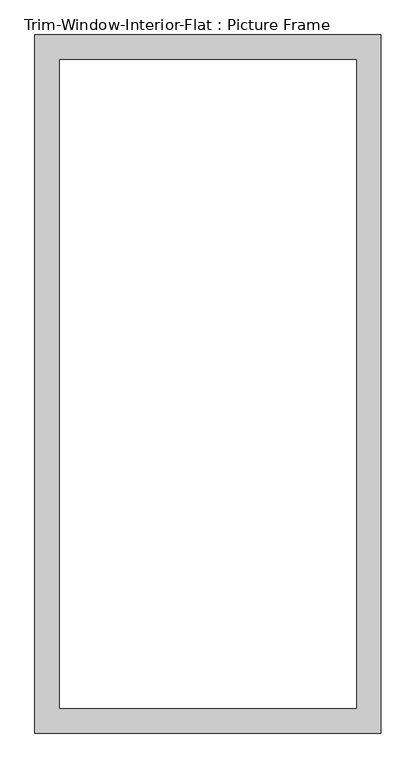
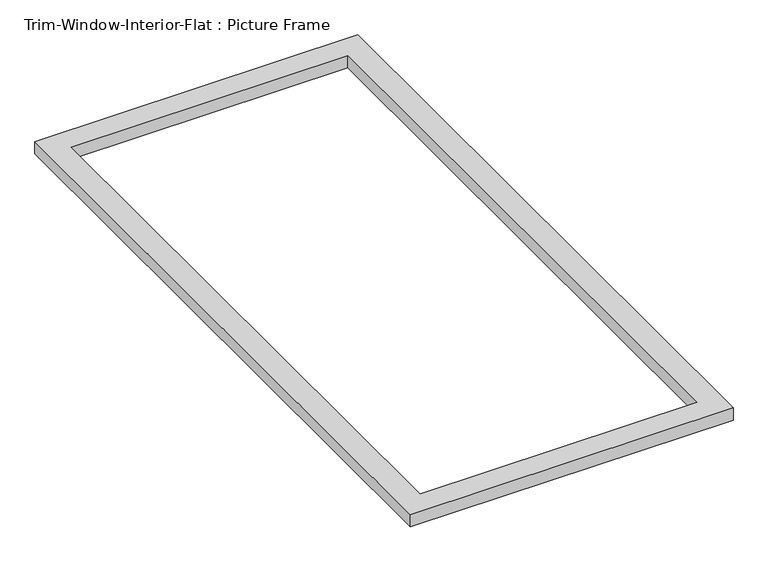
"""IFC4 building model written with IfcOpenShell, lengths in millimetres: proxy geometry, Trim-Window-Interior-Flat : Picture Frame."""

from ifc_helpers import new_model, si_unit, origin, origin_with_axes, place, context, project, spatial, polyline, outline, extrude, source, transform, mapped, element, save


def trim_window_interior_flat_picture_frame_b34e9b1a(model_context):
    return source(origin(), model_context, "Body", "SweptSolid", [
        extrude(outline(polyline([(400.05, 44.45), (400.05, -1568.45), (-400.05, -1568.45), (-400.05, 44.45), (400.05, 44.45)]), holes=[polyline([(342.9, -12.7), (-342.9, -12.7), (-342.9, -1511.3), (342.9, -1511.3), (342.9, -12.7)])]), origin_with_axes(), (0.0, 0.0, 1.0), 31.75),
    ])


if __name__ == "__main__":
    model = new_model("IFC4")
    model_context = context("Model", 3, world=origin())
    ifc_project = project(units=[si_unit("LENGTHUNIT", "METRE", prefix="MILLI")], contexts=[model_context])
    site = spatial("IfcSite", under=ifc_project)
    building = spatial("IfcBuilding", under=site)
    placement = place(None, origin())
    trim_window_interior_flat_picture_frame_shape = trim_window_interior_flat_picture_frame_b34e9b1a(model_context)
    element("IfcBuildingElementProxy", 1, Name="Trim-Window-Interior-Flat : Picture Frame", ObjectType="Trim-Window-Interior-Flat : Picture Frame", at=placement, inside=building, context=model_context, shape_type="MappedRepresentation", body=[
        mapped(trim_window_interior_flat_picture_frame_shape, transform((0.0, 0.0, 0.0), x_axis=(1.0, 0.0, 0.0), y_axis=(0.0, 1.0, 0.0), z_axis=(0.0, 0.0, 1.0))),
    ])
    save(model, "model.ifc")

# Revit data of these elements
# Type "Trim-Window-Interior-Flat : Picture Frame"
#   Trim Thickness_Picture Frame = 0' - 1 1/4"
#   Trim Width = 0' - 2 1/4"
#   Trim Thickness_with Sill = 0' - 0 3/4"
#   Sill Thickness = 0' - 1 1/4"
#   Opening Width [instance default] = 2' - 0"
#   Opening Height [instance default] = 3' - 0"
#   Default Elevation = 4' - 0"
#   Sill = no
#   Picture Frame = yes
#   Trim Material [instance default] = none
# Element 1 (IfcBuildingElementProxy, "Trim-Window-Interior-Flat : Picture Frame")
#   Opening Width = 2' - 4"
#   Opening Height = 5' - 0"
#   Trim Material = Wood - Stained
#   Materials on its faces: "Wood - Stained"
# Materials
#   "Wood - Stained": class "Wood", colour RGB 224 178 126, transparency 0, Cost = 0
